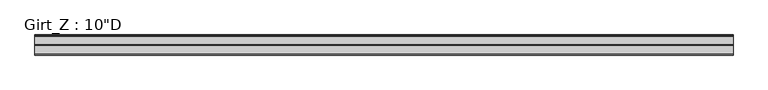
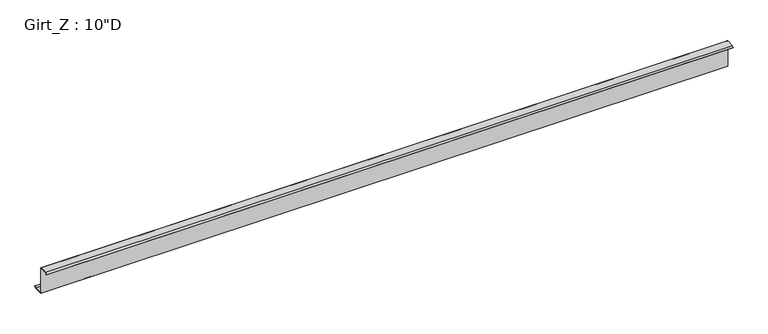
"""IFC4 building model written with IfcOpenShell, lengths in millimetres: beam geometry."""

from ifc_helpers import new_model, si_unit, point, frame, frame_2d, origin, place, context, project, spatial, polyline, circle_curve, trimmed, segment, composite_curve, outline, extrude, source, transform, mapped, element, save


def beam_3960b32e(model_context):
    return source(origin(), model_context, "Body", "SweptSolid", [
        extrude(outline(composite_curve([segment(polyline([(-77.9859375, 127.0), (-3.3734375, 127.0)]), True, "CONTINUOUS"), segment(trimmed(circle_curve(frame_2d((-3.3734375, 122.2375)), 4.7625), [point((-3.3734375, 127.0))], [point((1.3890625, 122.2375))], False, "CARTESIAN"), True, "CONTINUOUS"), segment(polyline([(1.3890625, 122.2375), (1.3890625, -122.2389339)]), True, "CONTINUOUS"), segment(trimmed(circle_curve(frame_2d((3.3748024, -122.2389339)), 1.9857399), [point((1.3890625, -122.2389339))], [point((3.2694106, -124.221875))], True, "CARTESIAN"), True, "CONTINUOUS"), segment(polyline([(3.2694106, -124.221875), (83.0404765, -124.221875), (94.4528742, -110.621109), (96.5810415, -112.4068534), (84.3359375, -127.0), (-1.3890625, -127.0), (-1.3890625, 122.2381931)]), True, "CONTINUOUS"), segment(trimmed(circle_curve(frame_2d((-3.3741066, 122.2381931)), 1.9850441), [point((-1.3890625, 122.2381931))], [point((-3.3005807, 124.221875))], True, "CARTESIAN"), True, "CONTINUOUS"), segment(polyline([(-3.3005807, 124.221875), (-76.6904765, 124.221875), (-88.1028742, 110.621109), (-90.2310415, 112.4068534), (-77.9859375, 127.0)]), True, "CONTINUOUS")], self_intersect=False)), frame((-3235.325, 0.0, 0.0), z_axis=(1.0, 0.0, 0.0), x_axis=(0.0, 1.0, 0.0)), (0.0, 0.0, 1.0), 6470.65),
    ])


if __name__ == "__main__":
    model = new_model("IFC4")
    model_context = context("Model", 3, world=origin())
    ifc_project = project(units=[si_unit("LENGTHUNIT", "METRE", prefix="MILLI")], contexts=[model_context])
    site = spatial("IfcSite", under=ifc_project)
    building = spatial("IfcBuilding", under=site)
    placement = place(None, origin())
    beam_shape = beam_3960b32e(model_context)
    element("IfcBeam", 1, ObjectType="Girt_Z : 10\"D", at=placement, inside=building, context=model_context, shape_type="MappedRepresentation", body=[
        mapped(beam_shape, transform((0.0, 0.0, 0.0), x_axis=(1.0, 0.0, 0.0), y_axis=(0.0, 1.0, 0.0), z_axis=(0.0, 0.0, 1.0))),
    ])
    save(model, "model.ifc")

# Revit data of these elements
# Type "Girt_Z : 10\"D"
#   half leg = 0' - 1 11/16"
#   Web_Thickness = 0' - 0 7/64"
#   Length [instance default] = 10' - 0"
#   Leg_2 = 0' - 3 3/8"
#   Leg_1 = 0' - 3 1/8"
#   Height = 0' - 10"
#   Structural Material [instance default] = none
# Element 1 (IfcBeam, "Girt_Z : 10\"D")
#   Structural Material = STRUCTURAL STEEL - SEE STRUCT. DWGS
#   Materials on its faces: "STRUCTURAL STEEL - SEE STRUCT. DWGS"
# Materials
#   "STRUCTURAL STEEL - SEE STRUCT. DWGS": class "Metal", colour RGB 137 146 153, transparency 0, Description = "Steel, mill finish", Cost = 0
